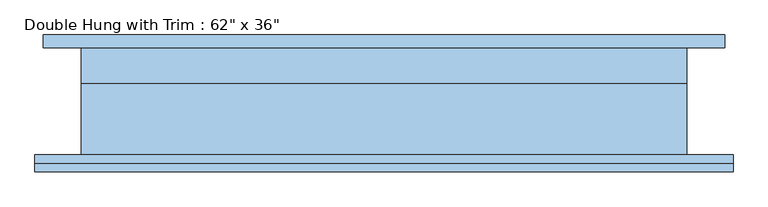
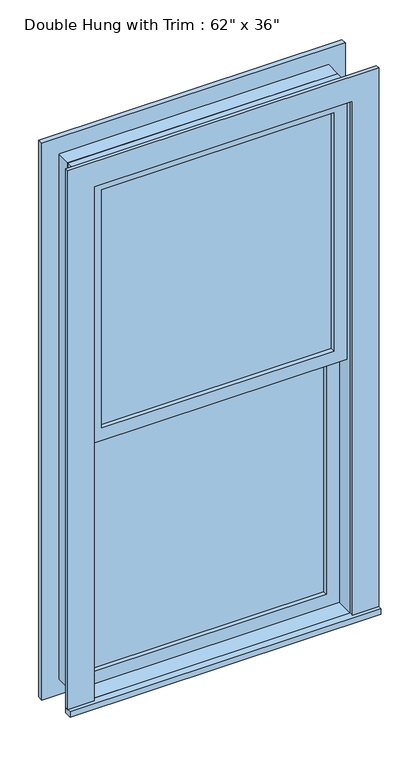
"""IFC4 building model written with IfcOpenShell, lengths in millimetres: window geometry."""

from ifc_helpers import new_model, si_unit, frame, origin, place, context, project, spatial, polyline, outline, extrude, source, transform, mapped, element, save


def window_86e2f1fd(model_context):
    return source(origin(), model_context, "Body", "SweptSolid", [
        extrude(outline(polyline([(-393.7, -1.5875), (-393.7, 11.1125), (393.7, 11.1125), (393.7, -1.5875), (-393.7, -1.5875)])), frame((0.0, 0.0, 571.5), z_axis=(0.0, 0.0, 1.0), x_axis=(1.0, 0.0, 0.0)), (0.0, 0.0, 1.0), 854.075),
        extrude(outline(polyline([(1470.025, -438.15), (527.05, -438.15), (527.05, 438.15), (1470.025, 438.15), (1470.025, -438.15)]), holes=[polyline([(1425.575, -393.7), (1425.575, 393.7), (571.5, 393.7), (571.5, -393.7), (1425.575, -393.7)])]), frame((0.0, -17.4625, 0.0), z_axis=(0.0, 1.0, 0.0), x_axis=(0.0, 0.0, 1.0)), (0.0, 0.0, 1.0), 44.45),
        extrude(outline(polyline([(-527.05, -106.3625), (-527.05, -80.9625), (527.05, -80.9625), (527.05, -106.3625), (-527.05, -106.3625)])), frame((0.0, 0.0, 508.0), z_axis=(0.0, 0.0, 1.0), x_axis=(1.0, 0.0, 0.0)), (0.0, 0.0, 1.0), 19.05),
        extrude(outline(polyline([(2368.55, -438.15), (2368.55, 438.15), (527.05, 438.15), (527.05, 527.05), (2457.45, 527.05), (2457.45, -527.05), (527.05, -527.05), (527.05, -438.15), (2368.55, -438.15)])), frame((0.0, -93.6625, 0.0), z_axis=(0.0, 1.0, 0.0), x_axis=(0.0, 0.0, 1.0)), (0.0, 0.0, 1.0), 12.7),
        extrude(outline(polyline([(2444.75, 514.35), (2444.75, -514.35), (450.85, -514.35), (450.85, 514.35), (2444.75, 514.35)]), holes=[polyline([(2355.85, 425.45), (539.75, 425.45), (539.75, -425.45), (2355.85, -425.45), (2355.85, 425.45)])]), frame((0.0, 80.9625, 0.0), z_axis=(0.0, 1.0, 0.0), x_axis=(0.0, 0.0, 1.0)), (0.0, 0.0, 1.0), 19.05),
        extrude(outline(polyline([(393.7, -33.3375), (393.7, -46.0375), (-393.7, -46.0375), (-393.7, -33.3375), (393.7, -33.3375)])), frame((0.0, 0.0, 1470.025), z_axis=(0.0, 0.0, 1.0), x_axis=(1.0, 0.0, 0.0)), (0.0, 0.0, 1.0), 854.075),
        extrude(outline(polyline([(2368.55, -438.15), (1425.575, -438.15), (1425.575, 438.15), (2368.55, 438.15), (2368.55, -438.15)]), holes=[polyline([(2324.1, -393.7), (2324.1, 393.7), (1470.025, 393.7), (1470.025, -393.7), (2324.1, -393.7)])]), frame((0.0, -61.9125, 0.0), z_axis=(0.0, 1.0, 0.0), x_axis=(0.0, 0.0, 1.0)), (0.0, 0.0, 1.0), 44.45),
        extrude(outline(polyline([(2387.6, -457.2), (508.0, -457.2), (508.0, 457.2), (2387.6, 457.2), (2387.6, -457.2)]), holes=[polyline([(2355.85, -425.45), (2355.85, 425.45), (539.75, 425.45), (539.75, -425.45), (2355.85, -425.45)])]), frame((0.0, 26.9875, 0.0), z_axis=(0.0, 1.0, 0.0), x_axis=(0.0, 0.0, 1.0)), (0.0, 0.0, 1.0), 53.975),
        extrude(outline(polyline([(2387.6, 457.2), (2387.6, -457.2), (508.0, -457.2), (508.0, 457.2), (2387.6, 457.2)]), holes=[polyline([(2368.55, 438.15), (527.05, 438.15), (527.05, -438.15), (2368.55, -438.15), (2368.55, 438.15)])]), frame((0.0, -80.9625, 0.0), z_axis=(0.0, 1.0, 0.0), x_axis=(0.0, 0.0, 1.0)), (0.0, 0.0, 1.0), 107.95),
    ])


if __name__ == "__main__":
    model = new_model("IFC4")
    model_context = context("Model", 3, world=origin())
    ifc_project = project(units=[si_unit("LENGTHUNIT", "METRE", prefix="MILLI")], contexts=[model_context])
    site = spatial("IfcSite", under=ifc_project)
    building = spatial("IfcBuilding", under=site)
    placement = place(None, origin())
    window_shape = window_86e2f1fd(model_context)
    element("IfcWindow", 1, ObjectType="Double Hung with Trim : 62\" x 36\"", at=placement, inside=building, context=model_context, shape_type="MappedRepresentation", body=[
        mapped(window_shape, transform((0.0, 0.0, 0.0), x_axis=(1.0, 0.0, 0.0), y_axis=(0.0, 1.0, 0.0), z_axis=(0.0, 0.0, 1.0))),
    ])
    save(model, "model.ifc")

# Revit data of these elements
# Type "Double Hung with Trim : 62\" x 36\""
#   Type Mark = "65"
#   COBie.Type.CreatedBy = "doug.wood@us.ibm.com"
#   COBie.Type.CreatedOn = "2016-04-14T02:07:26"
#   COBie.Type.Name = "Windows_Double Hung with Trim_62\" x 36\"_65"
#   COBie.Type.Category = "23-30 20 17 17 14 : Double-Hung Windows"
#   COBie.Type.Description = "Double Hung with Trim_62\" x 36\""
#   COBie.Type.Manufacturer = ""
#   COBie.Type.ModelNumber = ""
#   Construction Type Id = "GSP4R"
#   Assembly Code = "B2020100"
#   Analytic Construction = "1/8 in Pilkington single glazing"
#   COBie.Type.ReplacementCost = 0
#   Visual Light Transmittance = 0.9
#   Solar Heat Gain Coefficient = 0.78
#   Heat Transfer Coefficient (U) = 3.6886 W/(m²·K)
#   Height = 6' - 2"
#   Default Sill Height = 1' - 8"
#   Trim Projection - Ext. = 0' - 0 1/2"
#   Trim Projection - Int. = 0' - 0 3/4"
#   Trim Width - Exterior = 0' - 3 1/2"
#   Trim Width - Interior = 0' - 3 1/2"
#   Width = 3' - 0"
#   Window Inset = 0' - 0 3/4"
#   COBie.Type = no
#   Glass Pane Material = Glass
#   Sash Material = Sash - White
#   Trim Exterior Material = Trim - White
#   Trim Interior Material = Trim - White
#   Wall Closure = (empty or 0)
# Element 1 (IfcWindow, "Double Hung with Trim : 62\" x 36\"")
#   Materials on its faces: "Sash - White", "Trim - White", "Glass"
# Materials
#   "Glass": class "Glass", colour RGB 0 128 192, transparency 0.75, Description = "Soda Lime Glass", Cost = 0
#   "Sash - White": class "Wood", colour RGB 255 255 255, transparency 0, Cost = 0
#   "Trim - White": class "Wood", colour RGB 255 255 255, transparency 0, Cost = 0
